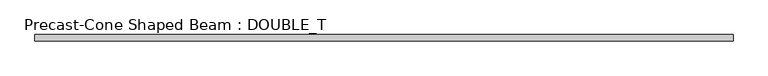
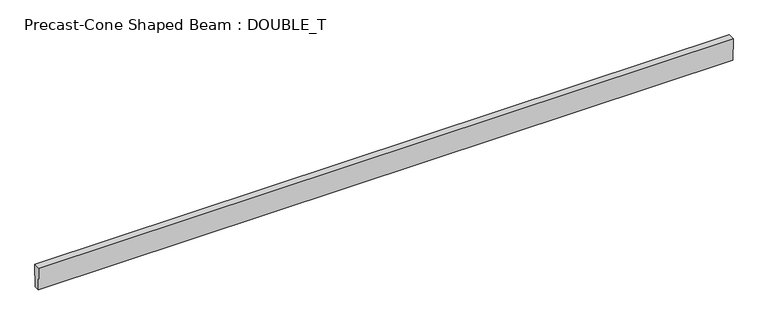
"""IFC4 building model written with IfcOpenShell, lengths in millimetres: beam geometry, Precast-Cone Shaped Beam : DOUBLE_T."""

from ifc_helpers import new_model, si_unit, frame, origin, place, context, project, spatial, polyline, outline, extrude, source, transform, mapped, element, save


def precast_cone_shaped_beam_double_t_b8a3e37e(model_context):
    return source(origin(), model_context, "Body", "SweptSolid", [
        extrude(outline(polyline([(50.8, -228.6), (-50.8, -228.6), (-63.5, 228.6), (63.5, 228.6), (50.8, -228.6)])), frame((-6727.03125, 0.0, 0.0), z_axis=(1.0, 0.0, 0.0), x_axis=(0.0, 1.0, 0.0)), (0.0, 0.0, 1.0), 13716.0),
    ])


if __name__ == "__main__":
    model = new_model("IFC4")
    model_context = context("Model", 3, world=origin())
    ifc_project = project(units=[si_unit("LENGTHUNIT", "METRE", prefix="MILLI")], contexts=[model_context])
    site = spatial("IfcSite", under=ifc_project)
    building = spatial("IfcBuilding", under=site)
    placement = place(None, origin())
    precast_cone_shaped_beam_double_t_shape = precast_cone_shaped_beam_double_t_b8a3e37e(model_context)
    element("IfcBeam", 1, ObjectType="Precast-Cone Shaped Beam : DOUBLE_T", at=placement, inside=building, context=model_context, shape_type="MappedRepresentation", body=[
        mapped(precast_cone_shaped_beam_double_t_shape, transform((0.0, 0.0, 0.0), x_axis=(1.0, 0.0, 0.0), y_axis=(0.0, 1.0, 0.0), z_axis=(0.0, 0.0, 1.0))),
    ])
    save(model, "model.ifc")

# Revit data of these elements
# Type "Precast-Cone Shaped Beam : DOUBLE_T"
#   Top Width = 0' - 5"
#   Tie Rod Weight [instance default] = 30
#   Tie Rod W [instance default] = 0.0660938 kip
#   Single Rebar Weight [instance default] = 50
#   Single Rebar W [instance default] = 0.110156 kip
#   Rebar Grids Weight [instance default] = 100
#   Rebar Grids W [instance default] = 0.220313 kip
#   Depth = 1' - 6"
#   Bottom Width = 0' - 4"
#   Length [instance default] = 5' - 0"
#   Structural Material [instance default] = Concrete, Precast
#   Assembly Code = ""
# Element 1 (IfcBeam, "Precast-Cone Shaped Beam : DOUBLE_T")
#   Length = 45' - 1 11/16"
#   Structural Material = Concrete - Precast Concrete - Normal Weight Concrete - 5 ksi
#   Materials on its faces: "Concrete - Precast Concrete - Normal Weight Concrete - 5 ksi"
# Materials
#   "Concrete, Precast": class "Concrete", colour RGB 198 187 187, transparency 0, Description = "Precast concrete", Cost = 0
#   "Concrete - Precast Concrete - Normal Weight Concrete - 5 ksi": class "Concrete", colour RGB 198 187 187, transparency 0, Cost = 0
